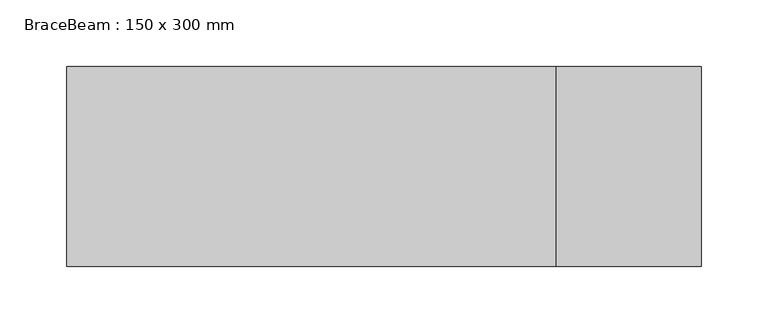
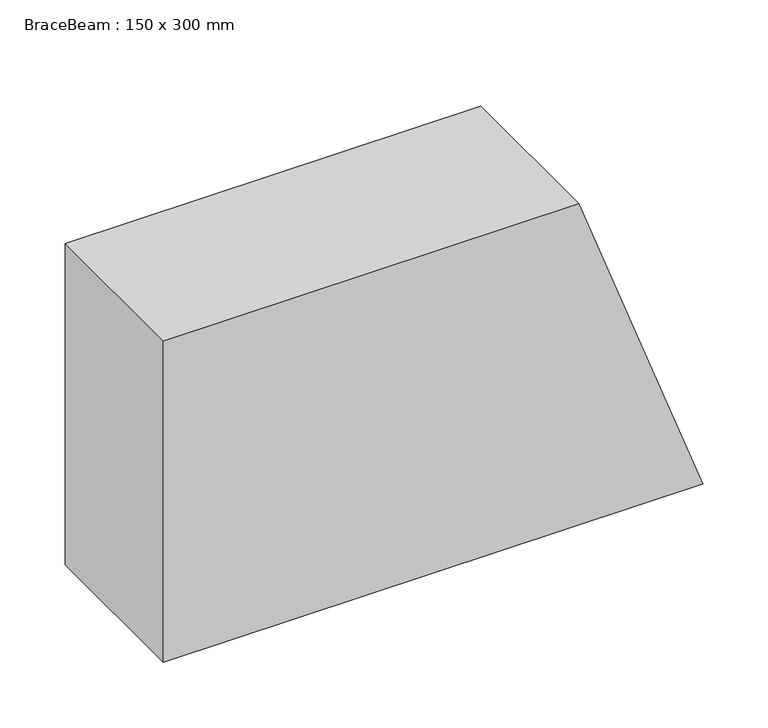
"""IFC4 building model written with IfcOpenShell, lengths in millimetres: beam geometry, BraceBeam : 150 x 300 mm."""

from ifc_helpers import new_model, si_unit, origin, place, context, project, spatial, faceted_brep, source, transform, mapped, element, save


def bracebeam_150_x_300_mm_189c702f(model_context):
    return source(origin(), model_context, "Body", "Brep", [
        faceted_brep([(-215.5051172, -75.0, -150.0), (-215.5051172, 75.0, -150.0), (260.4739864, 75.0, -150.0), (260.4739864, -75.0, -150.0), (-215.5051172, 75.0, 150.0), (151.2829162, 75.0, 150.0), (205.8784513, 75.0, 0.0), (-215.5051172, -75.0, 150.0), (151.2829162, -75.0, 150.0), (205.8784513, -75.0, 0.0)], [[[0, 1, 2, 3]], [[1, 4, 5, 6, 2]], [[4, 7, 8, 5]], [[7, 0, 3, 9, 8]], [[7, 4, 1, 0]], [[5, 8, 9, 3, 2, 6]]]),
    ])


if __name__ == "__main__":
    model = new_model("IFC4")
    model_context = context("Model", 3, world=origin())
    ifc_project = project(units=[si_unit("LENGTHUNIT", "METRE", prefix="MILLI")], contexts=[model_context])
    site = spatial("IfcSite", under=ifc_project)
    building = spatial("IfcBuilding", under=site)
    placement = place(None, origin())
    bracebeam_150_x_300_mm_shape = bracebeam_150_x_300_mm_189c702f(model_context)
    element("IfcBeam", 1, ObjectType="BraceBeam : 150 x 300 mm", at=placement, inside=building, context=model_context, shape_type="MappedRepresentation", body=[
        mapped(bracebeam_150_x_300_mm_shape, transform((0.0, 0.0, 0.0), x_axis=(1.0, 0.0, 0.0), y_axis=(0.0, 1.0, 0.0), z_axis=(0.0, 0.0, 1.0))),
    ])
    save(model, "model.ifc")

# Revit data of these elements
# Type "BraceBeam : 150 x 300 mm"
#   ExpertTruss = "Height\th\r\nWidth\tb"
#   Name [instance default] = ""
#   m [instance default] = 0 mm
#   ip_c_cut_control [instance default] = 1300 mm
#   ip_c_cut [instance default] = 1300 mm
#   h_fix [instance default] = 900 mm
#   d/2 [instance default] = 1750 mm
#   c_cut_incl [instance default] = -1000 mm
#   c_cut [instance default] = 0 mm
#   beta0_2 [instance default] = 90.00°
#   beta0_1 [instance default] = 90.00°
#   alfaMax [instance default] = 0.00°
#   alfa0_2 [instance default] = 90.00°
#   ZOffsetStr_0 [instance default] = 150 mm
#   ZOffsetStr [instance default] = 0 mm
#   ZOffsetEnd_0 [instance default] = 150 mm
#   ZOffsetEnd [instance default] = 0 mm
#   Beta2 [instance default] = 0.00°
#   Beta1 [instance default] = 0.00°
#   Alfa_str [instance default] = 0.00°
#   Alfa_cut_control [instance default] = 90.00°
#   Alfa_cut [instance default] = 90.00°
#   AlfaMAX [instance default] = 0.00°
#   Alfa2_0 [instance default] = 0.00°
#   Alfa2 [instance default] = 0.00°
#   Alfa1_0 [instance default] = 0.00°
#   Alfa1 [instance default] = 0.00°
#   A_max_Str [instance default] = 0.00°
#   h_void [instance default] = 3000 mm
#   beam_L_0 [instance default] = 100 mm
#   beam_L [instance default] = 0 mm
#   b_void [instance default] = 160 mm
#   alfa0_1 [instance default] = 90.00°
#   b = 150 mm
#   YOffsetStr [instance default] = 0 mm
#   YOffsetEnd [instance default] = 0 mm
#   XOffsetStr_0 [instance default] = 3500 mm
#   XOffsetStr [instance default] = 0 mm
#   XOffsetEnd_0 [instance default] = 3500 mm
#   XOffsetEnd [instance default] = 0 mm
#   L_void_0 [instance default] = 100 mm
#   L_void [instance default] = 0 mm
#   E2 [instance default] = 0.00°
#   E1 [instance default] = 0.00°
#   Length [instance default] = 3500 mm
#   h = 300 mm
#   Alfa [instance default] = 0.00°
#   A_max_End [instance default] = 0.00°
#   A_max [instance default] = 0.00°
#   A4 [instance default] = 0.00°
#   A3 [instance default] = 0.00°
#   A2 [instance default] = 0.00°
#   A1 [instance default] = 0.00°
#   BetaAngles [instance default] = no
#   Material [instance default] = Wood Standard
# Element 1 (IfcBeam, "BraceBeam : 150 x 300 mm")
#   d/2 = 369.84 mm
#   beta0_2 = 70.00°
#   alfaMax = -20.00°
#   alfa0_2 = 70.00°
#   AlfaMAX = -20.00°
#   Alfa2_0 = -20.00°
#   Alfa2 = -20.00°
#   h_void = 4091.911 mm
#   beam_L_0 = 873.529 mm
#   beam_L = 873.529 mm
#   XOffsetStr_0 = 589.68 mm
#   XOffsetStr = 150 mm
#   XOffsetEnd_0 = 580.054 mm
#   XOffsetEnd = 159.627 mm
#   L_void_0 = 2064.996 mm
#   L_void = 2064.996 mm
#   Materials on its faces: "Wood Standard"
# Materials
#   "Wood Standard": class "Drewno", colour RGB 196 146 67, transparency 0, Cost = 0
